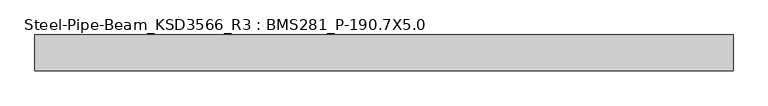
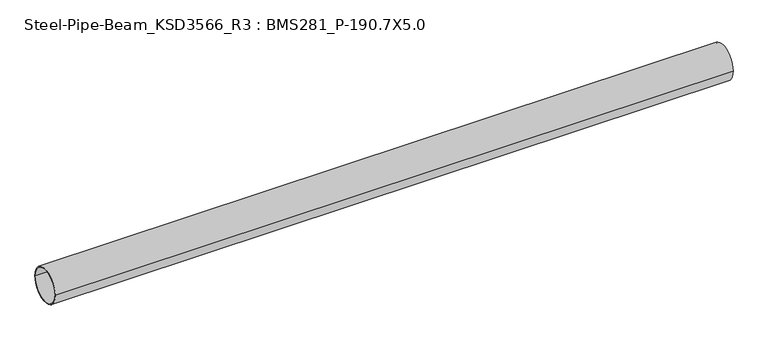
"""IFC4 building model written with IfcOpenShell, lengths in millimetres: member geometry, Steel-Pipe-Beam_KSD3566_R3 : BMS281_P-190.7X5.0."""

from ifc_helpers import new_model, si_unit, point, frame, origin, origin_2d, place, context, project, spatial, circle_curve, trimmed, segment, composite_curve, outline, extrude, source, transform, mapped, element, save


def steel_pipe_beam_ksd3566_r3_bms281_p_190_7x5_0_de5b040b(model_context):
    return source(origin(), model_context, "Body", "SweptSolid", [
        extrude(outline(composite_curve([segment(trimmed(circle_curve(origin_2d(), 95.35), [point((-95.35, 0.0))], [point((95.35, 0.0))], False, "CARTESIAN"), True, "CONTINUOUS"), segment(trimmed(circle_curve(origin_2d(), 95.35), [point((95.35, 0.0))], [point((-95.35, 0.0))], False, "CARTESIAN"), True, "CONTINUOUS")], self_intersect=False), holes=[composite_curve([segment(trimmed(circle_curve(origin_2d(), 90.35), [point((90.35, 0.0))], [point((-90.35, 0.0))], True, "CARTESIAN"), True, "CONTINUOUS"), segment(trimmed(circle_curve(origin_2d(), 90.35), [point((-90.35, 0.0))], [point((90.35, 0.0))], True, "CARTESIAN"), True, "CONTINUOUS")], self_intersect=False)]), frame((-1901.3396861, 0.0, 0.0), z_axis=(1.0, 0.0, 0.0), x_axis=(0.0, 1.0, 0.0)), (0.0, 0.0, 1.0), 3693.5342635),
    ])


if __name__ == "__main__":
    model = new_model("IFC4")
    model_context = context("Model", 3, world=origin())
    ifc_project = project(units=[si_unit("LENGTHUNIT", "METRE", prefix="MILLI")], contexts=[model_context])
    site = spatial("IfcSite", under=ifc_project)
    building = spatial("IfcBuilding", under=site)
    placement = place(None, origin())
    steel_pipe_beam_ksd3566_r3_bms281_p_190_7x5_0_shape = steel_pipe_beam_ksd3566_r3_bms281_p_190_7x5_0_de5b040b(model_context)
    element("IfcMember", 1, ObjectType="Steel-Pipe-Beam_KSD3566_R3 : BMS281_P-190.7X5.0", at=placement, inside=building, context=model_context, shape_type="MappedRepresentation", body=[
        mapped(steel_pipe_beam_ksd3566_r3_bms281_p_190_7x5_0_shape, transform((0.0, 0.0, 0.0), x_axis=(1.0, 0.0, 0.0), y_axis=(0.0, 1.0, 0.0), z_axis=(0.0, 0.0, 1.0))),
    ])
    save(model, "model.ifc")

# Revit data of these elements
# Type "Steel-Pipe-Beam_KSD3566_R3 : BMS281_P-190.7X5.0"
#   Keynote = "P-190.7X5.0"
#   SteelWeight = "Light"
#   t = 0.0050 m
#   Surface Area = 0.599102 m²/m
#   Section Area = 29.1697 cm²
#   Mass per Unit Length = 22.8982 kg/m
#   Length [instance default] = 1.5000 m
#   D = 0.1907 m
#   hec_material4 [instance default] = none
#   hec_material3 [instance default] = none
#   hec_material2 [instance default] = none
#   hec_material1 [instance default] = none
#   Structural Material [instance default] = Steel, 45-345
#   Assembly Code = ""
# Element 1 (IfcMember, "Steel-Pipe-Beam_KSD3566_R3 : BMS281_P-190.7X5.0")
#   Structural Material = none
# Materials
#   "Steel, 45-345": class "Metal", colour RGB 189 187 185, transparency 0, Description = "Steel 345 MPa", Cost = 0
